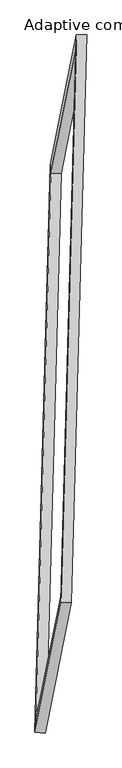
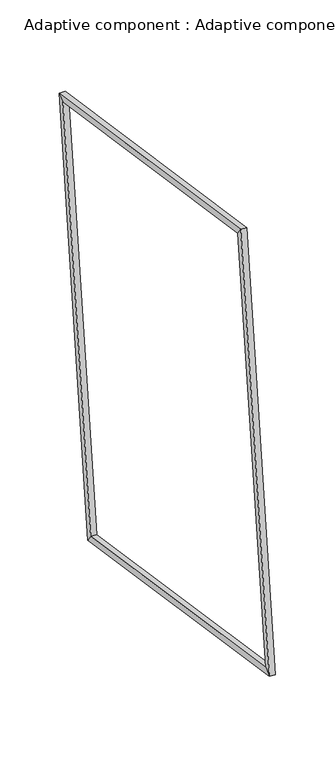
"""IFC4 building model written with IfcOpenShell, lengths in millimetres: proxy geometry, Adaptive component : Adaptive component."""

from ifc_helpers import new_model, si_unit, origin, place, context, project, spatial, faceted_brep, source, transform, mapped, element, save


def adaptive_component_adaptive_component_fe0fc2d4(model_context):
    return source(origin(), model_context, "Body", "Brep", [
        faceted_brep([(108.6112225, 1775.0157936, 3301.0047843), (173.6327454, 1774.9209813, 3300.4796603), (10.5099598, 956.5645185, -1257.0693988), (-54.3879249, 957.2796003, -1253.0899013), (106.3231212, 1699.5625796, 3248.5787039), (-52.1008479, 904.7791987, -1177.6883501), (171.3446441, 1699.4677673, 3248.0535798), (12.7970368, 904.0641169, -1181.6678475), (-87.6074219, -2617.6363648, -611.7717762), (-152.4104707, -2613.4666193, -608.4159947), (-146.6140313, -2538.1286494, -556.0947906), (-81.8109826, -2542.2983949, -559.4505721), (75.5153636, -1799.279902, 3945.7772829), (10.5886767, -1795.7304261, 3945.678691), (11.8099378, -1743.3452685, 3870.1722634), (76.7366248, -1746.8947445, 3870.2708553)], [[[0, 1, 2, 3]], [[4, 0, 3, 5]], [[6, 4, 5, 7]], [[1, 6, 7, 2]], [[3, 2, 8, 9]], [[5, 3, 9, 10]], [[7, 5, 10, 11]], [[2, 7, 11, 8]], [[9, 8, 12, 13]], [[10, 9, 13, 14]], [[11, 10, 14, 15]], [[8, 11, 15, 12]], [[13, 12, 1, 0]], [[14, 13, 0, 4]], [[15, 14, 4, 6]], [[12, 15, 6, 1]]]),
    ])


if __name__ == "__main__":
    model = new_model("IFC4")
    model_context = context("Model", 3, world=origin())
    ifc_project = project(units=[si_unit("LENGTHUNIT", "METRE", prefix="MILLI")], contexts=[model_context])
    site = spatial("IfcSite", under=ifc_project)
    building = spatial("IfcBuilding", under=site)
    placement = place(None, origin())
    adaptive_component_adaptive_component_shape = adaptive_component_adaptive_component_fe0fc2d4(model_context)
    element("IfcBuildingElementProxy", 1, Name="Adaptive component : Adaptive component", ObjectType="Adaptive component : Adaptive component", at=placement, inside=building, context=model_context, shape_type="MappedRepresentation", body=[
        mapped(adaptive_component_adaptive_component_shape, transform((0.0, 0.0, 0.0), x_axis=(1.0, 0.0, 0.0), y_axis=(0.0, 1.0, 0.0), z_axis=(0.0, 0.0, 1.0))),
    ])
    save(model, "model.ifc")

# Revit data of these elements
# Type "Adaptive component : Adaptive component"
#   r [instance default] = 2063.125 mm
#   2r [instance default] = 4126.251 mm
#   Number [instance default] = 5
#   Default Elevation = 0
# Element 1 (IfcBuildingElementProxy, "Adaptive component : Adaptive component")
#   r = 2850.439 mm
#   2r = 5700.877 mm
#   Number = 32
